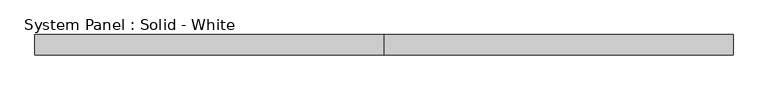
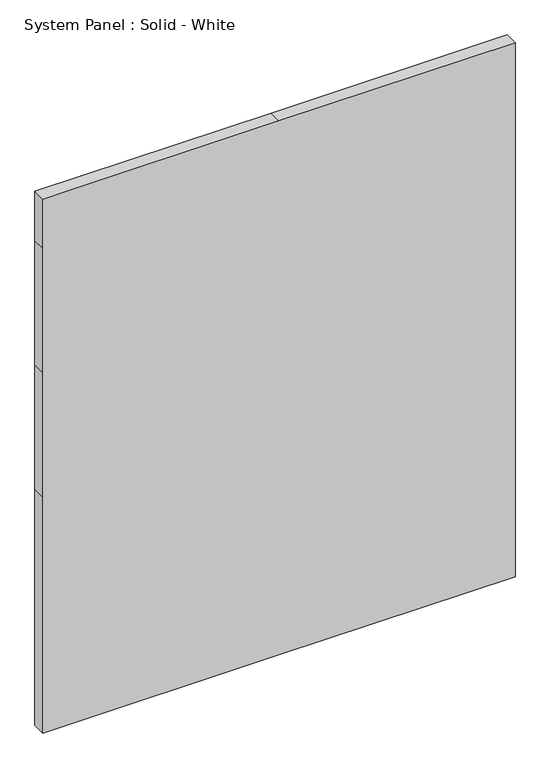
"""IFC4 building model written with IfcOpenShell, lengths in millimetres: plate geometry, System Panel : Solid - White."""

from ifc_helpers import new_model, si_unit, frame, origin, place, context, project, spatial, polyline, outline, extrude, source, transform, mapped, element, save


def system_panel_solid_white_63a197de(model_context):
    return source(origin(), model_context, "Body", "SweptSolid", [
        extrude(outline(polyline([(0.0, -1094.2054237), (0.0, 0.0), (0.0, 1094.2054237), (1155.7, 1094.2054237), (1765.3, 1094.2054237), (2374.9, 1094.2054237), (2616.2, 1094.2054237), (2616.2, 0.0), (2616.2, -1094.2054237), (2374.9, -1094.2054237), (1765.3, -1094.2054237), (1155.7, -1094.2054237), (0.0, -1094.2054237)])), frame((0.0, -44.45, 0.0), z_axis=(0.0, 1.0, 0.0), x_axis=(0.0, 0.0, 1.0)), (0.0, 0.0, 1.0), 63.5),
    ])


if __name__ == "__main__":
    model = new_model("IFC4")
    model_context = context("Model", 3, world=origin())
    ifc_project = project(units=[si_unit("LENGTHUNIT", "METRE", prefix="MILLI")], contexts=[model_context])
    site = spatial("IfcSite", under=ifc_project)
    building = spatial("IfcBuilding", under=site)
    placement = place(None, origin())
    system_panel_solid_white_shape = system_panel_solid_white_63a197de(model_context)
    element("IfcPlate", 1, ObjectType="System Panel : Solid - White", at=placement, inside=building, context=model_context, shape_type="MappedRepresentation", body=[
        mapped(system_panel_solid_white_shape, transform((0.0, 0.0, 0.0), x_axis=(1.0, 0.0, 0.0), y_axis=(0.0, 1.0, 0.0), z_axis=(0.0, 0.0, 1.0))),
    ])
    save(model, "model.ifc")

# Revit data of these elements
# Element 1 (IfcPlate, "System Panel : Solid - White")
#   Materials on its faces: "White Panel"
# Materials
#   "White Panel": class "Unassigned", colour RGB 255 255 255, transparency 0
